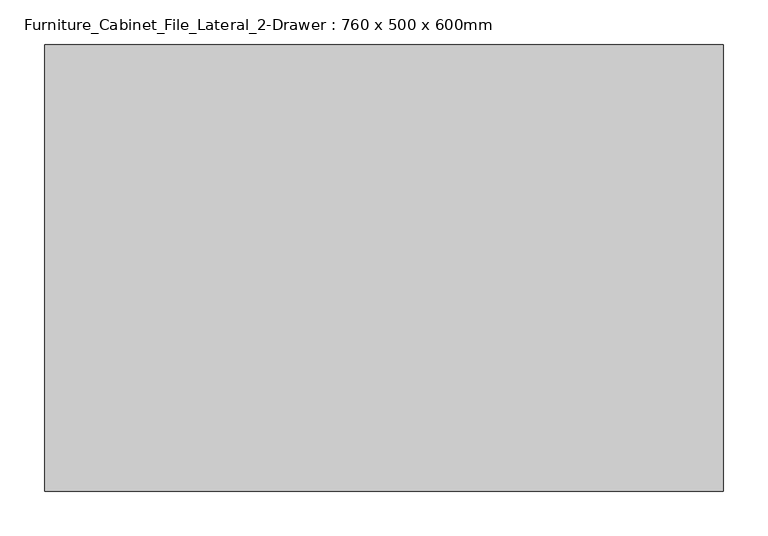
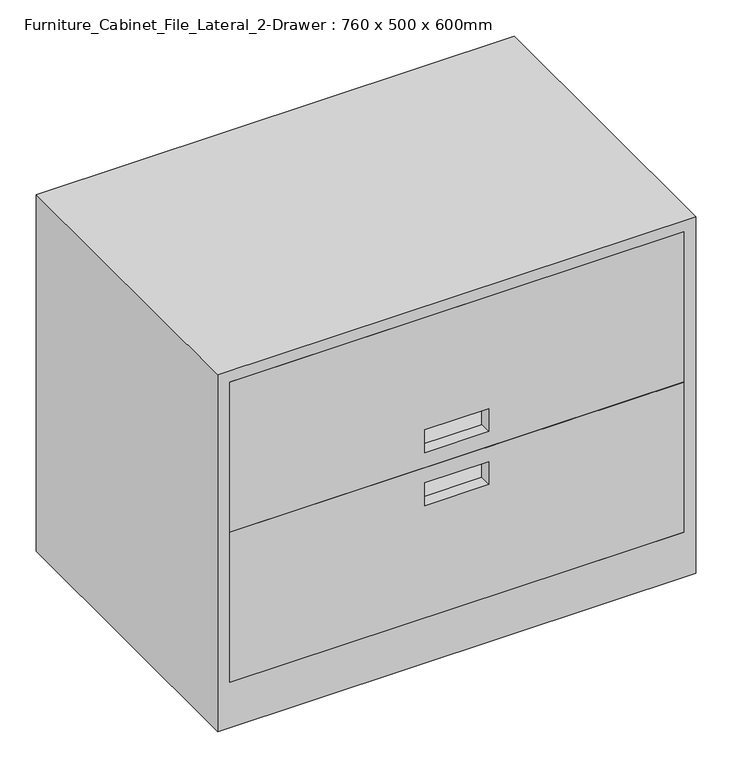
"""IFC4 building model written with IfcOpenShell, lengths in millimetres: furniture geometry, Furniture_Cabinet_File_Lateral_2-Drawer : 760 x 500 x 600mm."""

from ifc_helpers import new_model, si_unit, frame, origin, place, context, project, spatial, polyline, outline, extrude, faceted_brep, source, transform, mapped, element, save


def furniture_cabinet_file_lateral_2_drawer_760_x_500_x_600mm_44ef93b5(model_context):
    return source(origin(), model_context, "Body", "SolidModel", [
        extrude(outline(polyline([(76.2, -540.9725139), (76.2, 180.9274861), (328.575, 180.9274861), (328.575, -540.9725139), (76.2, -540.9725139)]), holes=[polyline([(303.175, -230.8225139), (303.175, -129.2225139), (265.075, -129.2225139), (265.075, -230.8225139), (303.175, -230.8225139)])]), frame((0.0, -1184.3183761, 0.0), z_axis=(0.0, 1.0, 0.0), x_axis=(0.0, 0.0, 1.0)), (0.0, 0.0, 1.0), 19.05),
        extrude(outline(polyline([(328.575, -540.9725139), (328.575, 180.9274861), (580.95, 180.9274861), (580.95, -540.9725139), (328.575, -540.9725139)]), holes=[polyline([(392.075, -230.8225139), (392.075, -129.2225139), (353.975, -129.2225139), (353.975, -230.8225139), (392.075, -230.8225139)])]), frame((0.0, -1184.3183761, 0.0), z_axis=(0.0, 1.0, 0.0), x_axis=(0.0, 0.0, 1.0)), (0.0, 0.0, 1.0), 19.05),
        faceted_brep([(199.9774861, -684.3183761, 600.0), (-560.0225139, -684.3183761, 600.0), (-560.0225139, -1184.3183761, 600.0), (199.9774861, -1184.3183761, 600.0), (199.9774861, -684.3183761, 0.0), (199.9774861, -1184.3183761, 0.0), (-560.0225139, -1184.3183761, 0.0), (-560.0225139, -684.3183761, 0.0), (180.9274861, -1184.3183761, 76.2), (-540.9725139, -1184.3183761, 76.2), (-540.9725139, -1184.3183761, 580.95), (180.9274861, -1184.3183761, 580.95), (-540.9725139, -703.3683761, 76.2), (180.9274861, -703.3683761, 76.2), (180.9274861, -703.3683761, 580.95), (-540.9725139, -703.3683761, 580.95)], [[[0, 1, 2, 3]], [[4, 5, 6, 7]], [[1, 0, 4, 7]], [[2, 1, 7, 6]], [[3, 2, 6, 5], [8, 9, 10, 11]], [[0, 3, 5, 4]], [[12, 13, 14, 15]], [[13, 12, 9, 8]], [[14, 13, 8, 11]], [[15, 14, 11, 10]], [[12, 15, 10, 9]]]),
    ])


if __name__ == "__main__":
    model = new_model("IFC4")
    model_context = context("Model", 3, world=origin())
    ifc_project = project(units=[si_unit("LENGTHUNIT", "METRE", prefix="MILLI")], contexts=[model_context])
    site = spatial("IfcSite", under=ifc_project)
    building = spatial("IfcBuilding", under=site)
    placement = place(None, origin())
    furniture_cabinet_file_lateral_2_drawer_760_x_500_x_600mm_shape = furniture_cabinet_file_lateral_2_drawer_760_x_500_x_600mm_44ef93b5(model_context)
    element("IfcFurniture", 1, ObjectType="Furniture_Cabinet_File_Lateral_2-Drawer : 760 x 500 x 600mm", at=placement, inside=building, context=model_context, shape_type="MappedRepresentation", body=[
        mapped(furniture_cabinet_file_lateral_2_drawer_760_x_500_x_600mm_shape, transform((0.0, 0.0, 0.0), x_axis=(1.0, 0.0, 0.0), y_axis=(0.0, 1.0, 0.0), z_axis=(0.0, 0.0, 1.0))),
    ])
    save(model, "model.ifc")

# Revit data of these elements
# Type "Furniture_Cabinet_File_Lateral_2-Drawer : 760 x 500 x 600mm"
#   Keynote = "N"
#   Depth = 500 mm
#   Height = 600 mm
#   Width = 760 mm
#   Material = Metal - Steel
#   Default Elevation = 0
#   Assembly Code = ""
# Element 1 (IfcFurniture, "Furniture_Cabinet_File_Lateral_2-Drawer : 760 x 500 x 600mm")
#   Materials on its faces: "Metal - Steel"
# Materials
#   "Metal - Steel": class "Metal", colour RGB 247 247 247, transparency 0
